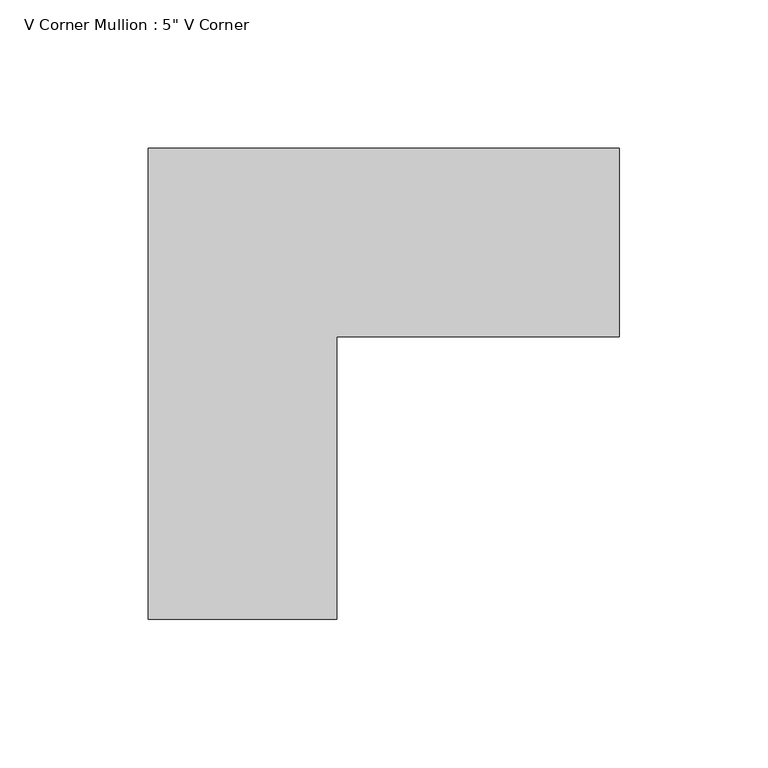
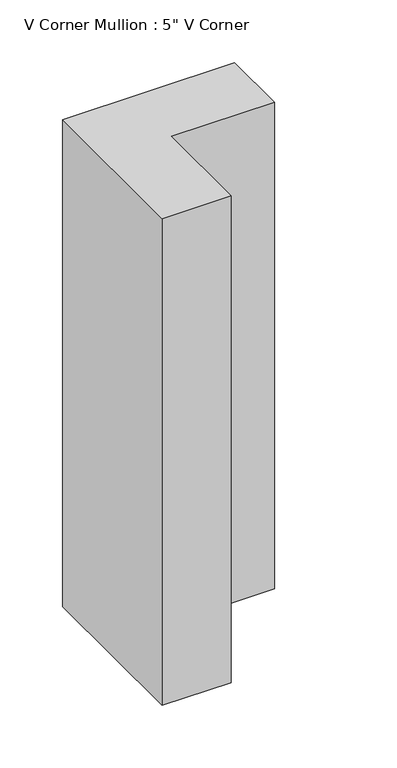
"""IFC4 building model written with IfcOpenShell, lengths in millimetres: member geometry."""

from ifc_helpers import new_model, si_unit, frame, origin, place, context, project, spatial, polyline, outline, extrude, source, transform, mapped, element, save


def member_9fe88380(model_context):
    return source(origin(), model_context, "Body", "SweptSolid", [
        extrude(outline(polyline([(63.5, 31.75), (-31.75, 31.75), (-31.75, -63.5), (-95.25, -63.5), (-95.25, 95.25), (63.5, 95.25), (63.5, 31.75)])), frame((0.0, 0.0, -474.1333333), z_axis=(0.0, 0.0, 1.0), x_axis=(1.0, 0.0, 0.0)), (0.0, 0.0, 1.0), 474.1333333),
    ])


if __name__ == "__main__":
    model = new_model("IFC4")
    model_context = context("Model", 3, world=origin())
    ifc_project = project(units=[si_unit("LENGTHUNIT", "METRE", prefix="MILLI")], contexts=[model_context])
    site = spatial("IfcSite", under=ifc_project)
    building = spatial("IfcBuilding", under=site)
    placement = place(None, origin())
    member_shape = member_9fe88380(model_context)
    element("IfcMember", 1, ObjectType="V Corner Mullion : 5\" V Corner", at=placement, inside=building, context=model_context, shape_type="MappedRepresentation", body=[
        mapped(member_shape, transform((0.0, 0.0, 0.0), x_axis=(1.0, 0.0, 0.0), y_axis=(0.0, 1.0, 0.0), z_axis=(0.0, 0.0, 1.0))),
    ])
    save(model, "model.ifc")

# Revit data of these elements
# Type "V Corner Mullion : 5\" V Corner"
#   built-in parameter 1007355 = 0.416667 (stored number, unit not read)
#   built-in parameter 1007354 = 0.416667 (stored number, unit not read)
#   built-in parameter 1007304 = 0.208333 (stored number, unit not read)
# Element 1 (IfcMember, "V Corner Mullion : 5\" V Corner")
#   Materials on its faces: "Aluminum"
# Materials
#   "Aluminum": class "Metal", colour RGB 244 245 246, transparency 0, Description = "Aluminum 6061", Cost = 0
